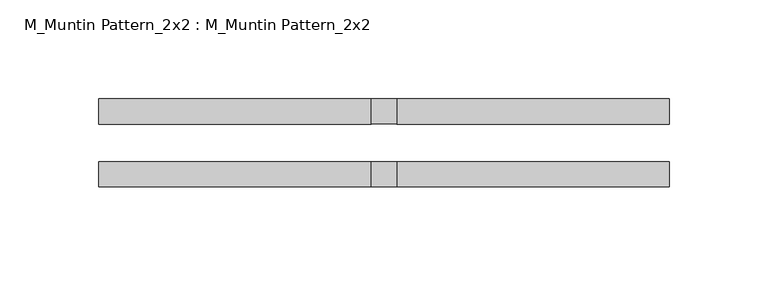
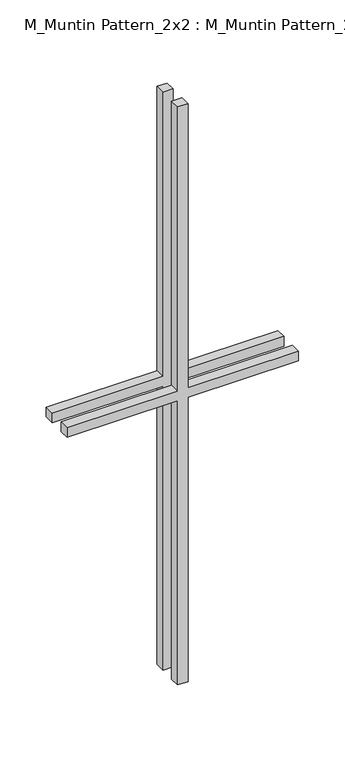
"""IFC4 building model written with IfcOpenShell, lengths in millimetres: proxy geometry, M_Muntin Pattern_2x2 : M_Muntin Pattern_2x2."""

import ifcopenshell
import ifcopenshell.guid

model = None  # the IFC model being written
_history = None  # IfcOwnerHistory: only IFC2X3 demands one
_inside = {}  # id of a spatial element -> (the spatial element, [elements in it])
_under = {}  # id of a project, library or spatial element -> (it, [spatial elements below it])
_declared = {}  # id of a project -> (the project, [libraries it declares])
_typed = {}  # id of a type object -> (the type object, [elements of that type])
_made_of = {}  # id of a material, layer set ... -> (it, [elements and type objects made of it])


def new_model(schema):
    """Start an empty IFC model of exactly this schema.

    Asked for "IFC4X3", IfcOpenShell would pick the latest addendum, in which some entities
    have other attributes; the version numbers below select the first issue.
    IFC2X3 requires an IfcOwnerHistory on every rooted entity: one is made here for all.
    """
    global model, _history
    if schema == "IFC4X3":
        model = ifcopenshell.file(schema_version=(4, 3, 0, 0))
    else:
        model = ifcopenshell.file(schema=schema)
    _inside.clear()
    _under.clear()
    _declared.clear()
    _typed.clear()
    _made_of.clear()
    _history = None
    if model.schema == "IFC2X3":
        org = make("IfcOrganization", Name="unknown")
        user = make(
            "IfcPersonAndOrganization",
            ThePerson=make("IfcPerson", FamilyName="unknown"),
            TheOrganization=org,
        )
        app = make(
            "IfcApplication",
            ApplicationDeveloper=org,
            Version="unknown",
            ApplicationFullName="unknown",
            ApplicationIdentifier="unknown",
        )
        _history = make(
            "IfcOwnerHistory",
            OwningUser=user,
            OwningApplication=app,
            ChangeAction="ADDED",
            CreationDate=0,
        )
    return model


def make(cls, **values):
    """One entity of the class cls with the attributes given. An attribute that is None is left unset."""
    return model.create_entity(
        cls, **{name: value for name, value in values.items() if value is not None}
    )


def rooted(cls, **values):
    """An entity with a GlobalId (a new one), such as an element, a storey or a relation."""
    return make(cls, GlobalId=ifcopenshell.guid.new(), OwnerHistory=_history, **values)


def si_unit(unit_type, name, prefix=None):
    """IfcSIUnit, for example si_unit("LENGTHUNIT", "METRE", prefix="MILLI")."""
    return make("IfcSIUnit", UnitType=unit_type, Prefix=prefix, Name=name)


def assignment(units):
    """IfcUnitAssignment: the units of a project."""
    return None if units is None else make("IfcUnitAssignment", Units=units)


def point(xyz):
    """IfcCartesianPoint."""
    return None if xyz is None else make("IfcCartesianPoint", Coordinates=xyz)


def direction(xyz):
    """IfcDirection."""
    return None if xyz is None else make("IfcDirection", DirectionRatios=xyz)


def frame(location, z_axis=None, x_axis=None):
    """IfcAxis2Placement3D, a coordinate frame: its origin and axes. An axis left out is left unset."""
    return make(
        "IfcAxis2Placement3D",
        Location=point(location),
        Axis=direction(z_axis),
        RefDirection=direction(x_axis),
    )


def origin():
    """The frame at (0, 0, 0) with its axes left unset."""
    return frame((0.0, 0.0, 0.0))


def place(relative_to, where):
    """IfcLocalPlacement: puts the frame where relative to a parent placement (None: the world)."""
    return make(
        "IfcLocalPlacement", PlacementRelTo=relative_to, RelativePlacement=where
    )


def context(
    kind, dimensions, precision=None, world=None, true_north=None, identifier=None
):
    """IfcGeometricRepresentationContext, for example the 3D "Model" context."""
    return make(
        "IfcGeometricRepresentationContext",
        ContextIdentifier=identifier,
        ContextType=kind,
        CoordinateSpaceDimension=dimensions,
        Precision=precision,
        WorldCoordinateSystem=world,
        TrueNorth=true_north,
    )


def project(units=None, contexts=None):
    """IfcProject with its units and contexts."""
    return rooted(
        "IfcProject",
        Name="project",
        RepresentationContexts=contexts,
        UnitsInContext=assignment(units),
    )


def spatial(cls, under=None, at=None, **own):
    """A site, building, storey or space (cls), placed at a placement, below another one or the project."""
    s = rooted(cls, ObjectPlacement=at, **own)
    if under is not None:
        _under.setdefault(under.id(), (under, []))[1].append(s)
    return s


def polyline(points):
    """IfcPolyline through the points."""
    return make("IfcPolyline", Points=[point(p) for p in points])


def outline(outer, holes=None, kind="AREA"):
    """IfcArbitraryClosedProfileDef: a profile drawn as a closed curve; with holes, ...WithVoids."""
    if holes is None:
        return make("IfcArbitraryClosedProfileDef", ProfileType=kind, OuterCurve=outer)
    return make(
        "IfcArbitraryProfileDefWithVoids",
        ProfileType=kind,
        OuterCurve=outer,
        InnerCurves=holes,
    )


def extrude(swept, where, along, depth):
    """IfcExtrudedAreaSolid: the profile swept, set in the frame where, extruded along a direction by depth."""
    return make(
        "IfcExtrudedAreaSolid",
        SweptArea=swept,
        Position=where,
        ExtrudedDirection=direction(along),
        Depth=depth,
    )


def shape(context_of_items, identifier, shape_type, items):
    """IfcShapeRepresentation: the items that make up one representation, for example the "Body"."""
    return make(
        "IfcShapeRepresentation",
        ContextOfItems=context_of_items,
        RepresentationIdentifier=identifier,
        RepresentationType=shape_type,
        Items=items,
    )


def source(mapping_origin, context_of_items, identifier, shape_type, items):
    """IfcRepresentationMap: a shape defined once, which mapped items show again and again."""
    return make(
        "IfcRepresentationMap",
        MappingOrigin=mapping_origin,
        MappedRepresentation=shape(context_of_items, identifier, shape_type, items),
    )


def transform(
    local_origin,
    x_axis=None,
    y_axis=None,
    z_axis=None,
    scale=None,
    scale2=None,
    scale3=None,
    uniform=True,
):
    """IfcCartesianTransformationOperator3D, or its non-uniform kind. x_axis, y_axis, z_axis: its Axis1, 2, 3."""
    if uniform:
        return make(
            "IfcCartesianTransformationOperator3D",
            Axis1=direction(x_axis),
            Axis2=direction(y_axis),
            LocalOrigin=point(local_origin),
            Scale=scale,
            Axis3=direction(z_axis),
        )
    return make(
        "IfcCartesianTransformationOperator3DnonUniform",
        Axis1=direction(x_axis),
        Axis2=direction(y_axis),
        LocalOrigin=point(local_origin),
        Scale=scale,
        Axis3=direction(z_axis),
        Scale2=scale2,
        Scale3=scale3,
    )


def mapped(mapping_source, mapping_target):
    """IfcMappedItem: shows the shape of a source again, moved by a transform."""
    return make(
        "IfcMappedItem", MappingSource=mapping_source, MappingTarget=mapping_target
    )


def made_of(thing, what):
    """Note that an element or type object is made of a material, layer set ...; save() writes the relation."""
    if what is not None:
        _made_of.setdefault(what.id(), (what, []))[1].append(thing)
    return thing


def element(
    cls,
    number,
    at=None,
    inside=None,
    cuts=None,
    type_object=None,
    material=None,
    context=None,
    identifier="Body",
    shape_type=None,
    held_by="IfcProductDefinitionShape",
    body=None,
    shapes=None,
    **own,
):
    """One element of the class cls, such as IfcWall. Its Tag is "e" and its number.

    at: its placement. inside: the storey or other place that contains it. cuts: it is an
    opening in that element (IfcRelVoidsElement). A single representation is given by context,
    identifier, shape_type and body (its items); several are given by shapes. held_by: the class
    of the entity that holds the representations. save() writes the other relations.
    """
    e = rooted(cls, Tag="e%d" % number, ObjectPlacement=at, **own)
    if body is not None:
        shapes = [shape(context, identifier, shape_type, body)]
    if shapes is not None:
        e.Representation = make(held_by, Representations=shapes)
    if inside is not None:
        _inside.setdefault(inside.id(), (inside, []))[1].append(e)
    if cuts is not None:
        rooted(
            "IfcRelVoidsElement", RelatingBuildingElement=cuts, RelatedOpeningElement=e
        )
    if type_object is not None:
        _typed.setdefault(type_object.id(), (type_object, []))[1].append(e)
    return made_of(e, material)


def aggregate(whole, parts):
    """IfcRelAggregates: a whole, such as a stair, and the parts it consists of."""
    return rooted("IfcRelAggregates", RelatingObject=whole, RelatedObjects=parts)


def save(model, path):
    """Write the relations noted so far, then the file.

    IfcRelAggregates (storeys below a building ...), IfcRelContainedInSpatialStructure (elements
    in a storey), IfcRelDefinesByType, IfcRelAssociatesMaterial and IfcRelDeclares: one each for
    every whole, place, type object, material and project.
    """
    for whole, parts in _under.values():
        aggregate(whole, parts)
    for where, things in _inside.values():
        rooted(
            "IfcRelContainedInSpatialStructure",
            RelatedElements=things,
            RelatingStructure=where,
        )
    for kind, things in _typed.values():
        rooted("IfcRelDefinesByType", RelatedObjects=things, RelatingType=kind)
    for what, things in _made_of.values():
        rooted("IfcRelAssociatesMaterial", RelatedObjects=things, RelatingMaterial=what)
    for by, libraries in _declared.values():
        rooted("IfcRelDeclares", RelatingContext=by, RelatedDefinitions=libraries)
    model.write(path)


def m_muntin_pattern_2x2_m_muntin_pattern_2x2_62480ac4(model_context):
    return source(origin(), model_context, "Body", "SweptSolid", [
        extrude(outline(polyline([(386.5, -6.35), (386.5, -144.2375), (373.8, -144.2375), (373.8, -6.35), (0.0, -6.35), (0.0, 6.35), (373.8, 6.35), (373.8, 144.2375), (386.5, 144.2375), (386.5, 6.35), (760.3, 6.35), (760.3, -6.35), (386.5, -6.35)])), frame((0.0, 9.525, 0.0), z_axis=(0.0, 1.0, 0.0), x_axis=(0.0, 0.0, 1.0)), (0.0, 0.0, 1.0), 12.7),
        extrude(outline(polyline([(386.5, -6.35), (386.5, -144.2375), (373.8, -144.2375), (373.8, -6.35), (0.0, -6.35), (0.0, 6.35), (373.8, 6.35), (373.8, 144.2375), (386.5, 144.2375), (386.5, 6.35), (760.3, 6.35), (760.3, -6.35), (386.5, -6.35)])), frame((0.0, -22.225, 0.0), z_axis=(0.0, 1.0, 0.0), x_axis=(0.0, 0.0, 1.0)), (0.0, 0.0, 1.0), 12.7),
    ])


if __name__ == "__main__":
    model = new_model("IFC4")
    model_context = context("Model", 3, world=origin())
    ifc_project = project(units=[si_unit("LENGTHUNIT", "METRE", prefix="MILLI")], contexts=[model_context])
    site = spatial("IfcSite", under=ifc_project)
    building = spatial("IfcBuilding", under=site)
    placement = place(None, origin())
    m_muntin_pattern_2x2_m_muntin_pattern_2x2_shape = m_muntin_pattern_2x2_m_muntin_pattern_2x2_62480ac4(model_context)
    element("IfcBuildingElementProxy", 1, Name="M_Muntin Pattern_2x2 : M_Muntin Pattern_2x2", ObjectType="M_Muntin Pattern_2x2 : M_Muntin Pattern_2x2", at=placement, inside=building, context=model_context, shape_type="MappedRepresentation", body=[
        mapped(m_muntin_pattern_2x2_m_muntin_pattern_2x2_shape, transform((0.0, 0.0, 0.0), x_axis=(1.0, 0.0, 0.0), y_axis=(0.0, 1.0, 0.0), z_axis=(0.0, 0.0, 1.0))),
    ])
    save(model, "model.ifc")

# Revit data of these elements
# Type "M_Muntin Pattern_2x2 : M_Muntin Pattern_2x2"
#   Width [instance default] = 120 cm
#   Thickness = 1.27 cm
#   Height [instance default] = 120 cm
#   Distance = 1.905 cm
#   Interior Material [instance default] = none
#   Exterior Material [instance default] = none
# Element 1 (IfcBuildingElementProxy, "M_Muntin Pattern_2x2 : M_Muntin Pattern_2x2")
#   Width = 28.8475 cm
#   Height = 76.03 cm
#   Interior Material = Wood - Stained
#   Exterior Material = Clad - White
#   Materials on its faces: "Clad - White", "Wood - Stained"
# Materials
#   "Clad - White": class "Wood", colour RGB 242 242 238, transparency 0, Cost = 0
#   "Wood - Stained": class "Wood", colour RGB 224 178 126, transparency 0, Cost = 0
